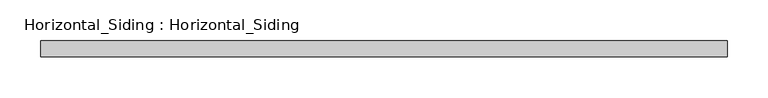
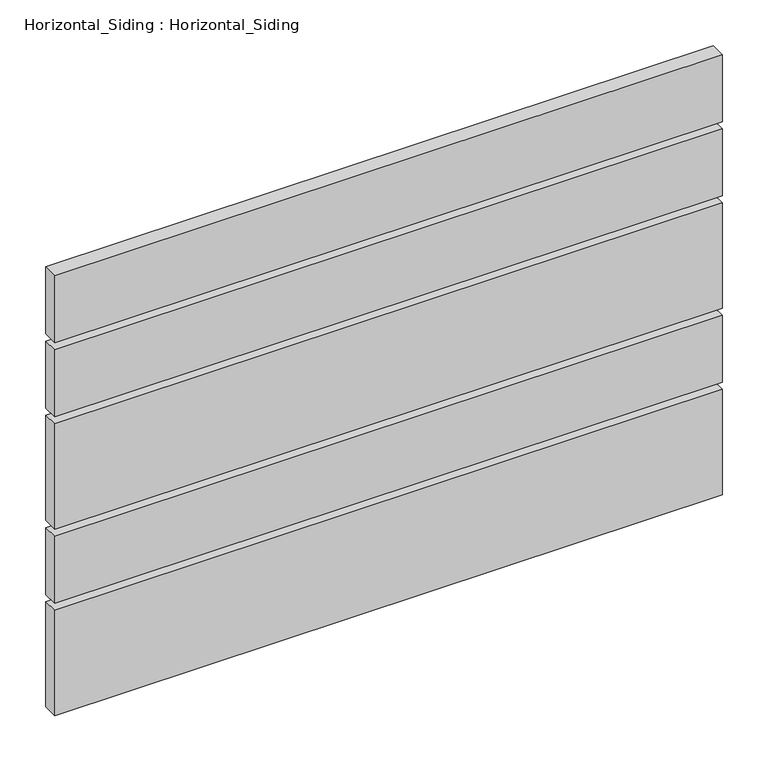
"""IFC4 building model written with IfcOpenShell, lengths in millimetres: plate geometry, Horizontal_Siding : Horizontal_Siding."""

from ifc_helpers import new_model, si_unit, frame, origin, place, context, project, spatial, polyline, outline, extrude, source, transform, mapped, element, save


def horizontal_siding_horizontal_siding_fcdd27e2(model_context):
    return source(origin(), model_context, "Body", "SweptSolid", [
        extrude(outline(polyline([(419.1, -19.05), (-419.1, -19.05), (-419.1, 0.0), (419.1, 0.0), (419.1, -19.05)])), frame((0.0, 0.0, 9.525), z_axis=(0.0, 0.0, 1.0), x_axis=(1.0, 0.0, 0.0)), (0.0, 0.0, 1.0), 139.7),
        extrude(outline(polyline([(419.1, -19.05), (-419.1, -19.05), (-419.1, 0.0), (419.1, 0.0), (419.1, -19.05)])), frame((0.0, 0.0, 158.75), z_axis=(0.0, 0.0, 1.0), x_axis=(1.0, 0.0, 0.0)), (0.0, 0.0, 1.0), 88.9),
        extrude(outline(polyline([(419.1, -19.05), (-419.1, -19.05), (-419.1, 0.0), (419.1, 0.0), (419.1, -19.05)])), frame((0.0, 0.0, 257.175), z_axis=(0.0, 0.0, 1.0), x_axis=(1.0, 0.0, 0.0)), (0.0, 0.0, 1.0), 139.7),
        extrude(outline(polyline([(419.1, -19.05), (-419.1, -19.05), (-419.1, 0.0), (419.1, 0.0), (419.1, -19.05)])), frame((0.0, 0.0, 406.4), z_axis=(0.0, 0.0, 1.0), x_axis=(1.0, 0.0, 0.0)), (0.0, 0.0, 1.0), 88.9),
        extrude(outline(polyline([(419.1, -19.05), (-419.1, -19.05), (-419.1, 0.0), (419.1, 0.0), (419.1, -19.05)])), frame((0.0, 0.0, 504.825), z_axis=(0.0, 0.0, 1.0), x_axis=(1.0, 0.0, 0.0)), (0.0, 0.0, 1.0), 88.9),
    ])


if __name__ == "__main__":
    model = new_model("IFC4")
    model_context = context("Model", 3, world=origin())
    ifc_project = project(units=[si_unit("LENGTHUNIT", "METRE", prefix="MILLI")], contexts=[model_context])
    site = spatial("IfcSite", under=ifc_project)
    building = spatial("IfcBuilding", under=site)
    placement = place(None, origin())
    horizontal_siding_horizontal_siding_shape = horizontal_siding_horizontal_siding_fcdd27e2(model_context)
    element("IfcPlate", 1, ObjectType="Horizontal_Siding : Horizontal_Siding", at=placement, inside=building, context=model_context, shape_type="MappedRepresentation", body=[
        mapped(horizontal_siding_horizontal_siding_shape, transform((0.0, 0.0, 0.0), x_axis=(1.0, 0.0, 0.0), y_axis=(0.0, 1.0, 0.0), z_axis=(0.0, 0.0, 1.0))),
    ])
    save(model, "model.ifc")

# Revit data of these elements
# Type "Horizontal_Siding : Horizontal_Siding"
#   Type Mark = "OUT"
#   Analytic Construction = "<None>"
#   extend = 0' - 2 3/4"
#   Width_2 = 0' - 3 1/2"
#   Width_1 = 0' - 5 1/2"
#   Gap = 0' - 0 3/8"
#   Plank Material = EXISTING HORZ. (1X4 & 1X6) WOOD SIDING (UNGROOVED PROFILE)
# Element 1 (IfcPlate, "Horizontal_Siding : Horizontal_Siding")
#   Materials on its faces: "EXISTING HORZ. (1X4 & 1X6) WOOD SIDING (UNGROOVED PROFILE)"
# Materials
#   "EXISTING HORZ. (1X4 & 1X6) WOOD SIDING (UNGROOVED PROFILE)": class "Wood", colour RGB 164 134 123, transparency 0, Description = "Pinus Echinata", Cost = 0
